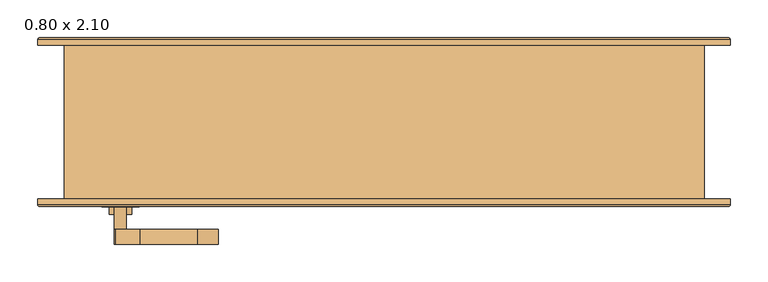
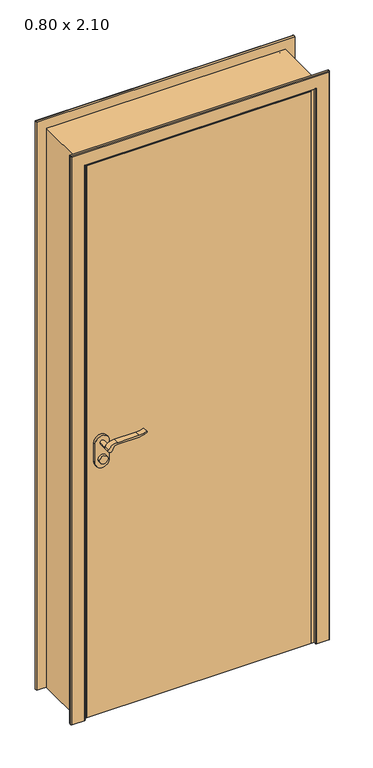
"""IFC4 building model written with IfcOpenShell, lengths in millimetres: door geometry, .CC_ND 300_PORTA SIMPLES DE ABRIR_COM EXTENSÃO : 0.80 x 2.10."""

from ifc_helpers import new_model, si_unit, point, frame, frame_2d, origin, origin_with_axes, place, context, project, spatial, polyline, circle_curve, ellipse_curve, trimmed, segment, composite_curve, outline, extrude, faceted_brep, source, transform, mapped, element, save
from ifc_brep_helpers import plane_surface, cylinder_surface, advanced_brep


def door_0_80_x_2_10_de608bb6(model_context):
    return source(origin(), model_context, "Body", "SolidModel", [
        extrude(outline(composite_curve([segment(trimmed(circle_curve(frame_2d((964.5, -350.0)), 15.0), [point((964.5, -335.0))], [point((964.5, -365.0))], False, "CARTESIAN"), True, "CONTINUOUS"), segment(trimmed(circle_curve(frame_2d((964.5, -350.0)), 15.0), [point((964.5, -365.0))], [point((964.5, -335.0))], False, "CARTESIAN"), True, "CONTINUOUS")], self_intersect=False)), frame((0.0, -137.9, 0.0), z_axis=(0.0, 1.0, 0.0), x_axis=(0.0, 0.0, 1.0)), (0.0, 0.0, 1.0), 10.0),
        extrude(outline(composite_curve([segment(trimmed(circle_curve(frame_2d((964.5, -350.0)), 15.0), [point((964.5, -335.0))], [point((964.5, -365.0))], False, "CARTESIAN"), True, "CONTINUOUS"), segment(trimmed(circle_curve(frame_2d((964.5, -350.0)), 15.0), [point((964.5, -365.0))], [point((964.5, -335.0))], False, "CARTESIAN"), True, "CONTINUOUS")], self_intersect=False)), frame((0.0, -77.9, 0.0), z_axis=(0.0, 1.0, 0.0), x_axis=(0.0, 0.0, 1.0)), (0.0, 0.0, 1.0), 10.0),
        extrude(outline(composite_curve([segment(trimmed(circle_curve(frame_2d((1024.5, -350.0)), 8.0), [point((1029.1523287, -356.5081363))], [point((1024.5, -342.0))], False, "CARTESIAN"), True, "CONTINUOUS"), segment(trimmed(circle_curve(frame_2d((1019.3738613, -324.6138099)), 18.1261387), [point((1024.5, -342.0))], [point((1037.5, -324.6138099))], True, "CARTESIAN"), True, "CONTINUOUS"), segment(polyline([(1037.5, -324.6138099), (1037.5, -248.3564091)]), True, "CONTINUOUS"), segment(trimmed(circle_curve(frame_2d((1096.7709207, -251.9396612)), 59.3791355), [point((1037.5, -248.3564091))], [point((1046.7135558, -220.0))], False, "CARTESIAN"), True, "CONTINUOUS"), segment(polyline([(1046.7135558, -220.0), (1049.5, -220.0)]), True, "CONTINUOUS"), segment(trimmed(circle_curve(frame_2d((1127.7850638, -248.4227909)), 83.2850902), [point((1049.5, -220.0))], [point((1044.5, -248.3564091))], True, "CARTESIAN"), True, "CONTINUOUS"), segment(polyline([(1044.5, -248.3564091), (1044.5, -324.6325667)]), True, "CONTINUOUS"), segment(trimmed(circle_curve(frame_2d((1007.2555521, -326.3324871)), 37.2832219), [point((1044.5, -324.6325667))], [point((1029.1523287, -356.5081363))], False, "CARTESIAN"), True, "CONTINUOUS")], self_intersect=False)), frame((0.0, -177.9, 0.0), z_axis=(0.0, 1.0, 0.0), x_axis=(0.0, 0.0, 1.0)), (0.0, 0.0, 1.0), 20.0),
        extrude(outline(composite_curve([segment(trimmed(circle_curve(frame_2d((1019.3738682, -324.6138122)), 18.1261318), [point((1024.4999903, -342.0))], [point((1037.5, -324.6138122))], True, "CARTESIAN"), True, "CONTINUOUS"), segment(polyline([(1037.5, -324.6138122), (1037.5, -248.3564091)]), True, "CONTINUOUS"), segment(trimmed(circle_curve(frame_2d((1096.7709207, -251.9396612)), 59.3791355), [point((1037.5, -248.3564091))], [point((1046.7135558, -220.0))], False, "CARTESIAN"), True, "CONTINUOUS"), segment(polyline([(1046.7135558, -220.0), (1049.5, -220.0)]), True, "CONTINUOUS"), segment(trimmed(circle_curve(frame_2d((1127.7850638, -248.4227909)), 83.2850902), [point((1049.5, -220.0))], [point((1044.5, -248.3564091))], True, "CARTESIAN"), True, "CONTINUOUS"), segment(polyline([(1044.5, -248.3564091), (1044.5, -324.6325667)]), True, "CONTINUOUS"), segment(trimmed(circle_curve(frame_2d((1007.2555521, -326.3324871)), 37.2832219), [point((1044.5, -324.6325667))], [point((1029.1523287, -356.5081363))], False, "CARTESIAN"), True, "CONTINUOUS"), segment(trimmed(circle_curve(frame_2d((1024.5, -350.0)), 8.0), [point((1029.1523287, -356.5081363))], [point((1024.4999903, -342.0))], False, "CARTESIAN"), True, "CONTINUOUS")], self_intersect=False)), frame((0.0, -47.9, 0.0), z_axis=(0.0, 1.0, 0.0), x_axis=(0.0, 0.0, 1.0)), (0.0, 0.0, 1.0), 20.0),
        extrude(outline(composite_curve([segment(trimmed(circle_curve(frame_2d((1024.5, -350.0)), 8.0), [point((1024.5, -342.0))], [point((1024.5, -358.0))], False, "CARTESIAN"), True, "CONTINUOUS"), segment(trimmed(circle_curve(frame_2d((1024.5, -350.0)), 8.0), [point((1024.5, -358.0))], [point((1024.5, -342.0))], False, "CARTESIAN"), True, "CONTINUOUS")], self_intersect=False)), frame((0.0, -157.9, 0.0), z_axis=(0.0, 1.0, 0.0), x_axis=(0.0, 0.0, 1.0)), (0.0, 0.0, 1.0), 30.0),
        extrude(outline(composite_curve([segment(trimmed(circle_curve(frame_2d((1024.5, -350.0)), 8.0), [point((1024.5, -342.0))], [point((1024.5, -358.0))], False, "CARTESIAN"), True, "CONTINUOUS"), segment(trimmed(circle_curve(frame_2d((1024.5, -350.0)), 8.0), [point((1024.5, -358.0))], [point((1024.5, -342.0))], False, "CARTESIAN"), True, "CONTINUOUS")], self_intersect=False)), frame((0.0, -77.9, 0.0), z_axis=(0.0, 1.0, 0.0), x_axis=(0.0, 0.0, 1.0)), (0.0, 0.0, 1.0), 30.0),
        extrude(outline(composite_curve([segment(trimmed(circle_curve(frame_2d((954.5, -350.0)), 25.0), [point((954.5, -375.0))], [point((954.5, -325.0))], False, "CARTESIAN"), True, "CONTINUOUS"), segment(polyline([(954.5, -325.0), (1024.5, -325.0)]), True, "CONTINUOUS"), segment(trimmed(circle_curve(frame_2d((1024.5, -350.0)), 25.0), [point((1024.5, -325.0))], [point((1024.5, -375.0))], False, "CARTESIAN"), True, "CONTINUOUS"), segment(polyline([(1024.5, -375.0), (954.5, -375.0)]), True, "CONTINUOUS")], self_intersect=False)), frame((0.0, -127.9, 0.0), z_axis=(0.0, 1.0, 0.0), x_axis=(0.0, 0.0, 1.0)), (0.0, 0.0, 1.0), 10.0),
        extrude(outline(composite_curve([segment(trimmed(circle_curve(frame_2d((954.5, -350.0)), 25.0), [point((954.5, -375.0))], [point((954.5, -325.0))], False, "CARTESIAN"), True, "CONTINUOUS"), segment(polyline([(954.5, -325.0), (1024.5, -325.0)]), True, "CONTINUOUS"), segment(trimmed(circle_curve(frame_2d((1024.5, -350.0)), 25.0), [point((1024.5, -325.0))], [point((1024.5, -375.0))], False, "CARTESIAN"), True, "CONTINUOUS"), segment(polyline([(1024.5, -375.0), (954.5, -375.0)]), True, "CONTINUOUS")], self_intersect=False)), frame((0.0, -87.9, 0.0), z_axis=(0.0, 1.0, 0.0), x_axis=(0.0, 0.0, 1.0)), (0.0, 0.0, 1.0), 10.0),
        advanced_brep(
        [(-460.0, -117.9, 0.0), (-410.0, -117.9, 0.0), (-410.0, -124.9, 0.0), (-413.0, -127.9, 0.0), (-457.0, -127.9, 0.0), (-460.0, -124.9, 0.0), (-460.0, -117.9, 2135.0), (460.0, -117.9, 2135.0), (460.0, -117.9, 0.0), (410.0, -117.9, 0.0), (410.0, -117.9, 2085.0), (-410.0, -117.9, 2085.0), (-410.0, -124.9, 2085.0), (-413.0, -127.9, 2088.0), (413.0, -127.9, 2088.0), (413.0, -127.9, 0.0), (457.0, -127.9, 0.0), (457.0, -127.9, 2132.0), (-457.0, -127.9, 2132.0), (-460.0, -124.9, 2135.0), (460.0, -124.9, 2135.0), (460.0, -124.9, 0.0), (410.0, -124.9, 0.0), (410.0, -124.9, 2085.0)],
        [
            (0, 1),
            (1, 2),
            (2, 3, circle_curve(frame((-413.0, -124.9, 0.0), z_axis=(0.0, 0.0, -1.0), x_axis=(1.0, 0.0, 0.0)), 3.0)),
            (3, 4),
            (4, 5, circle_curve(frame((-457.0, -124.9, 0.0), z_axis=(0.0, 0.0, -1.0), x_axis=(1.0, 0.0, 0.0)), 3.0)),
            (5, 0),
            (0, 6),
            (6, 7),
            (7, 8),
            (8, 9),
            (9, 10),
            (10, 11),
            (11, 1),
            (11, 12),
            (12, 2),
            (12, 13, ellipse_curve(frame((-413.0, -124.9, 2088.0), z_axis=(-0.7071067811865475, 0.0, -0.7071067811865475), x_axis=(0.7071067811865474, 0.0, -0.7071067811865476)), 4.2426407, 3.0)),
            (13, 3),
            (13, 14),
            (14, 15),
            (15, 16),
            (16, 17),
            (17, 18),
            (18, 4),
            (18, 19, ellipse_curve(frame((-457.0, -124.9, 2132.0), z_axis=(-0.7071067811865475, 0.0, -0.7071067811865475), x_axis=(0.7071067811865474, 0.0, -0.7071067811865476)), 4.2426407, 3.0)),
            (19, 5),
            (19, 6),
            (7, 20),
            (20, 21),
            (21, 8),
            (21, 16, circle_curve(frame((457.0, -124.9, 0.0), z_axis=(0.0, 0.0, -1.0), x_axis=(-1.0, 0.0, 0.0)), 3.0)),
            (15, 22, circle_curve(frame((413.0, -124.9, 0.0), z_axis=(0.0, 0.0, -1.0), x_axis=(-1.0, 0.0, 0.0)), 3.0)),
            (22, 9),
            (23, 10),
            (22, 23),
            (14, 23, ellipse_curve(frame((413.0, -124.9, 2088.0), z_axis=(0.7071067811865475, 0.0, -0.7071067811865475), x_axis=(0.7071067811865474, 0.0, 0.7071067811865476)), 4.2426407, 3.0)),
            (20, 17, ellipse_curve(frame((457.0, -124.9, 2132.0), z_axis=(0.7071067811865475, 0.0, -0.7071067811865475), x_axis=(0.7071067811865474, 0.0, 0.7071067811865476)), 4.2426407, 3.0)),
            (23, 12),
            (19, 20),
        ],
        [
            plane_surface(frame((-410.0, -117.9, 0.0), z_axis=(0.0, 0.0, -1.0), x_axis=(0.0, 1.0, 0.0))),
            plane_surface(frame((-460.0, -117.9, 0.0), z_axis=(0.0, 1.0, 0.0), x_axis=(0.0, 0.0, 1.0))),
            plane_surface(frame((-410.0, -117.9, 0.0), z_axis=(1.0, 0.0, 0.0), x_axis=(0.0, 0.0, 1.0))),
            cylinder_surface(frame((-413.0, -124.9, 0.0), z_axis=(0.0, 0.0, -1.0), x_axis=(1.0, 0.0, 0.0)), 3.0),
            plane_surface(frame((-413.0, -127.9, 0.0), z_axis=(0.0, -1.0, 0.0), x_axis=(0.0, 0.0, 1.0))),
            cylinder_surface(frame((-457.0, -124.9, 0.0), z_axis=(0.0, 0.0, -1.0), x_axis=(1.0, 0.0, 0.0)), 3.0),
            plane_surface(frame((-460.0, -124.9, 0.0), z_axis=(-1.0, 0.0, 0.0), x_axis=(0.0, 0.0, 1.0))),
            plane_surface(frame((460.0, -124.9, 2135.0), z_axis=(1.0, 0.0, 0.0), x_axis=(0.0, 0.0, -1.0))),
            plane_surface(frame((410.0, -117.9, 0.0), z_axis=(0.0, 0.0, -1.0), x_axis=(0.0, 1.0, 0.0))),
            plane_surface(frame((410.0, -117.9, 2085.0), z_axis=(-1.0, 0.0, 0.0), x_axis=(0.0, 0.0, -1.0))),
            cylinder_surface(frame((413.0, -124.9, 2085.0), z_axis=(0.0, 0.0, 1.0), x_axis=(-1.0, 0.0, 0.0)), 3.0),
            cylinder_surface(frame((457.0, -124.9, 2085.0), z_axis=(0.0, 0.0, 1.0), x_axis=(-1.0, 0.0, 0.0)), 3.0),
            plane_surface(frame((-410.0, -117.9, 2085.0), z_axis=(0.0, 0.0, -1.0), x_axis=(1.0, 0.0, 0.0))),
            plane_surface(frame((-460.0, -124.9, 2135.0), z_axis=(0.0, 0.0, 1.0), x_axis=(1.0, 0.0, 0.0))),
            cylinder_surface(frame((-410.0, -124.9, 2088.0), z_axis=(-1.0, 0.0, 0.0), x_axis=(0.0, 0.0, -1.0)), 3.0),
            cylinder_surface(frame((-410.0, -124.9, 2132.0), z_axis=(-1.0, 0.0, 0.0), x_axis=(0.0, 0.0, -1.0)), 3.0),
        ],
        [
            (0, [[1, 2, 3, 4, 5, 6]]),
            (1, [[-1, 7, 8, 9, 10, 11, 12, 13]]),
            (2, [[-2, -13, 14, 15]]),
            (3, [[-3, -15, 16, 17]]),
            (4, [[-4, -17, 18, 19, 20, 21, 22, 23]]),
            (5, [[-5, -23, 24, 25]]),
            (6, [[-6, -25, 26, -7]]),
            (7, [[27, 28, 29, -9]]),
            (8, [[-29, 30, -20, 31, 32, -10]]),
            (9, [[33, -11, -32, 34]]),
            (10, [[35, -34, -31, -19]]),
            (11, [[36, -21, -30, -28]]),
            (12, [[-14, -12, -33, 37]]),
            (13, [[-26, 38, -27, -8]]),
            (14, [[-16, -37, -35, -18]]),
            (15, [[-24, -22, -36, -38]]),
        ],
    ),
        advanced_brep(
        [(460.0, 86.9, 0.0), (410.0, 86.9, 0.0), (410.0, 93.9157283, 0.0), (412.9842717, 96.9, 0.0), (457.0342217, 96.9, 0.0), (460.0, 93.9342217, 0.0), (460.0, 86.9, 2135.0), (-460.0, 86.9, 2135.0), (-460.0, 86.9, 0.0), (-410.0, 86.9, 0.0), (-410.0, 86.9, 2085.0), (410.0, 86.9, 2085.0), (410.0, 93.9157283, 2085.0), (412.9842717, 96.9, 2087.9842717), (-412.9842717, 96.9, 2087.9842717), (-412.9842717, 96.9, 0.0), (-457.0342217, 96.9, 0.0), (-457.0342217, 96.9, 2132.0342217), (457.0342217, 96.9, 2132.0342217), (460.0, 93.9342217, 2135.0), (-460.0, 93.9342217, 2135.0), (-460.0, 93.9342217, 0.0), (-410.0, 93.9157283, 0.0), (-410.0, 93.9157283, 2085.0)],
        [
            (0, 1),
            (1, 2),
            (2, 3, circle_curve(frame((412.9842717, 93.9157283, 0.0), z_axis=(0.0, 0.0, -1.0), x_axis=(1.0, 0.0, 0.0)), 2.9842717)),
            (3, 4),
            (4, 5, circle_curve(frame((457.0342217, 93.9342217, 0.0), z_axis=(0.0, 0.0, -1.0), x_axis=(1.0, 0.0, 0.0)), 2.9657783)),
            (5, 0),
            (0, 6),
            (6, 7),
            (7, 8),
            (8, 9),
            (9, 10),
            (10, 11),
            (11, 1),
            (11, 12),
            (12, 2),
            (12, 13, ellipse_curve(frame((412.9842717, 93.9157283, 2087.9842717), z_axis=(0.7071067811865475, 0.0, -0.7071067811865475), x_axis=(-0.7071067811865474, 0.0, -0.7071067811865476)), 4.2203975, 2.9842717)),
            (13, 3),
            (13, 14),
            (14, 15),
            (15, 16),
            (16, 17),
            (17, 18),
            (18, 4),
            (18, 19, ellipse_curve(frame((457.0342217, 93.9342217, 2132.0342217), z_axis=(0.7071067811865475, 0.0, -0.7071067811865475), x_axis=(-0.7071067811865474, 0.0, -0.7071067811865476)), 4.1942438, 2.9657783)),
            (19, 5),
            (19, 6),
            (7, 20),
            (20, 21),
            (21, 8),
            (21, 16, circle_curve(frame((-457.0342217, 93.9342217, 0.0), z_axis=(0.0, 0.0, -1.0), x_axis=(-1.0, 0.0, 0.0)), 2.9657783)),
            (15, 22, circle_curve(frame((-412.9842717, 93.9157283, 0.0), z_axis=(0.0, 0.0, -1.0), x_axis=(-1.0, 0.0, 0.0)), 2.9842717)),
            (22, 9),
            (23, 10),
            (22, 23),
            (14, 23, ellipse_curve(frame((-412.9842717, 93.9157283, 2087.9842717), z_axis=(-0.7071067811865475, 0.0, -0.7071067811865475), x_axis=(-0.7071067811865474, 0.0, 0.7071067811865476)), 4.2203975, 2.9842717)),
            (20, 17, ellipse_curve(frame((-457.0342217, 93.9342217, 2132.0342217), z_axis=(-0.7071067811865475, 0.0, -0.7071067811865475), x_axis=(-0.7071067811865474, 0.0, 0.7071067811865476)), 4.1942438, 2.9657783)),
            (23, 12),
            (19, 20),
        ],
        [
            plane_surface(frame((410.0, 86.9, 0.0), z_axis=(0.0, 0.0, -1.0), x_axis=(0.0, 1.0, 0.0))),
            plane_surface(frame((460.0, 86.9, 0.0), z_axis=(0.0, -1.0, 0.0), x_axis=(0.0, 0.0, 1.0))),
            plane_surface(frame((410.0, 86.9, 0.0), z_axis=(-1.0, 0.0, 0.0), x_axis=(0.0, 0.0, 1.0))),
            cylinder_surface(frame((412.9842717, 93.9157283, 0.0), z_axis=(0.0, 0.0, -1.0), x_axis=(1.0, 0.0, 0.0)), 2.9842717),
            plane_surface(frame((412.9842717, 96.9, 0.0), z_axis=(0.0, 1.0, 0.0), x_axis=(0.0, 0.0, 1.0))),
            cylinder_surface(frame((457.0342217, 93.9342217, 0.0), z_axis=(0.0, 0.0, -1.0), x_axis=(1.0, 0.0, 0.0)), 2.9657783),
            plane_surface(frame((460.0, 93.9342217, 0.0), z_axis=(1.0, 0.0, 0.0), x_axis=(0.0, 0.0, 1.0))),
            plane_surface(frame((-460.0, 93.9342217, 2135.0), z_axis=(-1.0, 0.0, 0.0), x_axis=(0.0, 0.0, -1.0))),
            plane_surface(frame((-410.0, 86.9, 0.0), z_axis=(0.0, 0.0, -1.0), x_axis=(0.0, 1.0, 0.0))),
            plane_surface(frame((-410.0, 86.9, 2085.0), z_axis=(1.0, 0.0, 0.0), x_axis=(0.0, 0.0, -1.0))),
            cylinder_surface(frame((-412.9842717, 93.9157283, 2085.0), z_axis=(0.0, 0.0, 1.0), x_axis=(-1.0, 0.0, 0.0)), 2.9842717),
            cylinder_surface(frame((-457.0342217, 93.9342217, 2085.0), z_axis=(0.0, 0.0, 1.0), x_axis=(-1.0, 0.0, 0.0)), 2.9657783),
            plane_surface(frame((410.0, 86.9, 2085.0), z_axis=(0.0, 0.0, -1.0), x_axis=(-1.0, 0.0, 0.0))),
            plane_surface(frame((460.0, 93.9342217, 2135.0), z_axis=(0.0, 0.0, 1.0), x_axis=(-1.0, 0.0, 0.0))),
            cylinder_surface(frame((410.0, 93.9157283, 2087.9842717), z_axis=(1.0, 0.0, 0.0), x_axis=(0.0, 0.0, 1.0)), 2.9842717),
            cylinder_surface(frame((410.0, 93.9342217, 2132.0342217), z_axis=(1.0, 0.0, 0.0), x_axis=(0.0, 0.0, 1.0)), 2.9657783),
        ],
        [
            (0, [[1, 2, 3, 4, 5, 6]]),
            (1, [[-1, 7, 8, 9, 10, 11, 12, 13]]),
            (2, [[-2, -13, 14, 15]]),
            (3, [[-3, -15, 16, 17]]),
            (4, [[-4, -17, 18, 19, 20, 21, 22, 23]]),
            (5, [[-5, -23, 24, 25]]),
            (6, [[-6, -25, 26, -7]]),
            (7, [[27, 28, 29, -9]]),
            (8, [[-29, 30, -20, 31, 32, -10]]),
            (9, [[33, -11, -32, 34]]),
            (10, [[35, -34, -31, -19]]),
            (11, [[36, -21, -30, -28]]),
            (12, [[-14, -12, -33, 37]]),
            (13, [[-26, 38, -27, -8]]),
            (14, [[-16, -37, -35, -18]]),
            (15, [[-24, -22, -36, -38]]),
        ],
    ),
        faceted_brep([(392.0, 86.9, 0.0), (425.0, 86.9, 0.0), (425.0, -117.9, 0.0), (400.0, -117.9, 0.0), (400.0, -87.9, 0.0), (392.0, -87.9, 0.0), (392.0, 86.9, 2067.0), (-392.0, 86.9, 2067.0), (-392.0, 86.9, 0.0), (-425.0, 86.9, 0.0), (-425.0, 86.9, 2100.0), (425.0, 86.9, 2100.0), (425.0, -117.9, 2100.0), (-425.0, -117.9, 2100.0), (-425.0, -117.9, 0.0), (-400.0, -117.9, 0.0), (-400.0, -117.9, 2075.0), (400.0, -117.9, 2075.0), (400.0, -87.9, 2075.0), (-400.0, -87.9, 2075.0), (-400.0, -87.9, 0.0), (-392.0, -87.9, 0.0), (-392.0, -87.9, 2067.0), (392.0, -87.9, 2067.0)], [[[0, 1, 2, 3, 4, 5]], [[1, 0, 6, 7, 8, 9, 10, 11]], [[2, 1, 11, 12]], [[3, 2, 12, 13, 14, 15, 16, 17]], [[4, 3, 17, 18]], [[5, 4, 18, 19, 20, 21, 22, 23]], [[0, 5, 23, 6]], [[7, 22, 21, 8]], [[8, 21, 20, 15, 14, 9]], [[13, 10, 9, 14]], [[19, 16, 15, 20]], [[12, 11, 10, 13]], [[18, 17, 16, 19]], [[6, 23, 22, 7]]]),
        extrude(outline(polyline([(-400.0, -87.9), (400.0, -87.9), (400.0, -117.9), (-400.0, -117.9), (-400.0, -87.9)])), origin_with_axes(), (0.0, 0.0, 1.0), 2075.0),
    ])


if __name__ == "__main__":
    model = new_model("IFC4")
    model_context = context("Model", 3, world=origin())
    ifc_project = project(units=[si_unit("LENGTHUNIT", "METRE", prefix="MILLI")], contexts=[model_context])
    site = spatial("IfcSite", under=ifc_project)
    building = spatial("IfcBuilding", under=site)
    placement = place(None, origin())
    door_0_80_x_2_10_shape = door_0_80_x_2_10_de608bb6(model_context)
    element("IfcDoor", 1, ObjectType=".CC_ND 300_PORTA SIMPLES DE ABRIR_COM EXTENSÃO : 0.80 x 2.10", at=placement, inside=building, context=model_context, shape_type="MappedRepresentation", body=[
        mapped(door_0_80_x_2_10_shape, transform((0.0, 0.0, 0.0), x_axis=(1.0, 0.0, 0.0), y_axis=(0.0, 1.0, 0.0), z_axis=(0.0, 0.0, 1.0))),
    ])
    save(model, "model.ifc")

# Revit data of these elements
# Type ".CC_ND 300_PORTA SIMPLES DE ABRIR_COM EXTENSÃO : 0.80 x 2.10"
#   Type Mark = "153"
#   Rough Width = 0.85 m
#   Espessura moldura externa = 0.01 m
#   Espessura moldura interna = 0.01 m
#   Largura moldura = 0.05 m
#   Extensão acabamento exterior [instance default] = 0.00 m
#   Extensão acabamento interior [instance default] = 0.00 m
#   Espessura batente = 0.025 m
#   Thickness = 0.03 m
#   Altura batente = 2.085 m
#   Aux Arco [instance default] = 0.80 m
#   Rough Height = 2.125 m
#   Height = 2.10 m
#   Width = 0.80 m
#   Moldura interna [instance default] = yes
#   Moldura externa [instance default] = yes
#   Porta = .MADEIRA COM PINTURA ESMALTE BRANCO ACETINADO
#   Moldura = .MADEIRA COM PINTURA ESMALTE BRANCO ACETINADO
#   Maçaneta = .ALUMÍNIO
#   Batente = .MADEIRA COM PINTURA ESMALTE BRANCO ACETINADO
#   Function = (empty or 0)
#   Wall Closure = (empty or 0)
# Element 1 (IfcDoor, ".CC_ND 300_PORTA SIMPLES DE ABRIR_COM EXTENSÃO : 0.80 x 2.10")
#   Extensão acabamento interior = 0.031 m
#   Aux Arco = 0.831 m
#   Materials on its faces: ".MADEIRA COM PINTURA ESMALTE BRANCO ACETINADO", ".ALUMÍNIO"
# Materials
#   ".MADEIRA COM PINTURA ESMALTE BRANCO ACETINADO": class ".CC_MADEIRAS", colour RGB 240 240 240, transparency 0, Description = "Madeira com pintura esmalte branco acetinado.", Cost = 0
#   ".ALUMÍNIO": class "CC_METAIS", colour RGB 244 244 244, transparency 0, Description = "Material alumínio", Cost = 0
